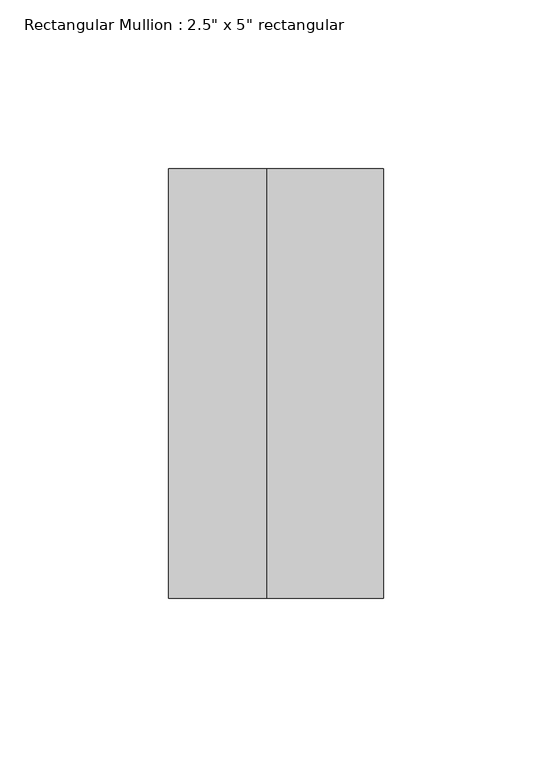
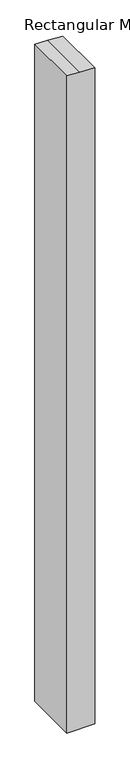
"""IFC4 building model written with IfcOpenShell, lengths in millimetres: member geometry."""

import ifcopenshell
import ifcopenshell.guid

model = None  # the IFC model being written
_history = None  # IfcOwnerHistory: only IFC2X3 demands one
_inside = {}  # id of a spatial element -> (the spatial element, [elements in it])
_under = {}  # id of a project, library or spatial element -> (it, [spatial elements below it])
_declared = {}  # id of a project -> (the project, [libraries it declares])
_typed = {}  # id of a type object -> (the type object, [elements of that type])
_made_of = {}  # id of a material, layer set ... -> (it, [elements and type objects made of it])


def new_model(schema):
    """Start an empty IFC model of exactly this schema.

    Asked for "IFC4X3", IfcOpenShell would pick the latest addendum, in which some entities
    have other attributes; the version numbers below select the first issue.
    IFC2X3 requires an IfcOwnerHistory on every rooted entity: one is made here for all.
    """
    global model, _history
    if schema == "IFC4X3":
        model = ifcopenshell.file(schema_version=(4, 3, 0, 0))
    else:
        model = ifcopenshell.file(schema=schema)
    _inside.clear()
    _under.clear()
    _declared.clear()
    _typed.clear()
    _made_of.clear()
    _history = None
    if model.schema == "IFC2X3":
        org = make("IfcOrganization", Name="unknown")
        user = make(
            "IfcPersonAndOrganization",
            ThePerson=make("IfcPerson", FamilyName="unknown"),
            TheOrganization=org,
        )
        app = make(
            "IfcApplication",
            ApplicationDeveloper=org,
            Version="unknown",
            ApplicationFullName="unknown",
            ApplicationIdentifier="unknown",
        )
        _history = make(
            "IfcOwnerHistory",
            OwningUser=user,
            OwningApplication=app,
            ChangeAction="ADDED",
            CreationDate=0,
        )
    return model


def make(cls, **values):
    """One entity of the class cls with the attributes given. An attribute that is None is left unset."""
    return model.create_entity(
        cls, **{name: value for name, value in values.items() if value is not None}
    )


def rooted(cls, **values):
    """An entity with a GlobalId (a new one), such as an element, a storey or a relation."""
    return make(cls, GlobalId=ifcopenshell.guid.new(), OwnerHistory=_history, **values)


def si_unit(unit_type, name, prefix=None):
    """IfcSIUnit, for example si_unit("LENGTHUNIT", "METRE", prefix="MILLI")."""
    return make("IfcSIUnit", UnitType=unit_type, Prefix=prefix, Name=name)


def assignment(units):
    """IfcUnitAssignment: the units of a project."""
    return None if units is None else make("IfcUnitAssignment", Units=units)


def point(xyz):
    """IfcCartesianPoint."""
    return None if xyz is None else make("IfcCartesianPoint", Coordinates=xyz)


def direction(xyz):
    """IfcDirection."""
    return None if xyz is None else make("IfcDirection", DirectionRatios=xyz)


def frame(location, z_axis=None, x_axis=None):
    """IfcAxis2Placement3D, a coordinate frame: its origin and axes. An axis left out is left unset."""
    return make(
        "IfcAxis2Placement3D",
        Location=point(location),
        Axis=direction(z_axis),
        RefDirection=direction(x_axis),
    )


def origin():
    """The frame at (0, 0, 0) with its axes left unset."""
    return frame((0.0, 0.0, 0.0))


def place(relative_to, where):
    """IfcLocalPlacement: puts the frame where relative to a parent placement (None: the world)."""
    return make(
        "IfcLocalPlacement", PlacementRelTo=relative_to, RelativePlacement=where
    )


def context(
    kind, dimensions, precision=None, world=None, true_north=None, identifier=None
):
    """IfcGeometricRepresentationContext, for example the 3D "Model" context."""
    return make(
        "IfcGeometricRepresentationContext",
        ContextIdentifier=identifier,
        ContextType=kind,
        CoordinateSpaceDimension=dimensions,
        Precision=precision,
        WorldCoordinateSystem=world,
        TrueNorth=true_north,
    )


def project(units=None, contexts=None):
    """IfcProject with its units and contexts."""
    return rooted(
        "IfcProject",
        Name="project",
        RepresentationContexts=contexts,
        UnitsInContext=assignment(units),
    )


def spatial(cls, under=None, at=None, **own):
    """A site, building, storey or space (cls), placed at a placement, below another one or the project."""
    s = rooted(cls, ObjectPlacement=at, **own)
    if under is not None:
        _under.setdefault(under.id(), (under, []))[1].append(s)
    return s


def polyline(points):
    """IfcPolyline through the points."""
    return make("IfcPolyline", Points=[point(p) for p in points])


def outline(outer, holes=None, kind="AREA"):
    """IfcArbitraryClosedProfileDef: a profile drawn as a closed curve; with holes, ...WithVoids."""
    if holes is None:
        return make("IfcArbitraryClosedProfileDef", ProfileType=kind, OuterCurve=outer)
    return make(
        "IfcArbitraryProfileDefWithVoids",
        ProfileType=kind,
        OuterCurve=outer,
        InnerCurves=holes,
    )


def extrude(swept, where, along, depth):
    """IfcExtrudedAreaSolid: the profile swept, set in the frame where, extruded along a direction by depth."""
    return make(
        "IfcExtrudedAreaSolid",
        SweptArea=swept,
        Position=where,
        ExtrudedDirection=direction(along),
        Depth=depth,
    )


def shape(context_of_items, identifier, shape_type, items):
    """IfcShapeRepresentation: the items that make up one representation, for example the "Body"."""
    return make(
        "IfcShapeRepresentation",
        ContextOfItems=context_of_items,
        RepresentationIdentifier=identifier,
        RepresentationType=shape_type,
        Items=items,
    )


def source(mapping_origin, context_of_items, identifier, shape_type, items):
    """IfcRepresentationMap: a shape defined once, which mapped items show again and again."""
    return make(
        "IfcRepresentationMap",
        MappingOrigin=mapping_origin,
        MappedRepresentation=shape(context_of_items, identifier, shape_type, items),
    )


def transform(
    local_origin,
    x_axis=None,
    y_axis=None,
    z_axis=None,
    scale=None,
    scale2=None,
    scale3=None,
    uniform=True,
):
    """IfcCartesianTransformationOperator3D, or its non-uniform kind. x_axis, y_axis, z_axis: its Axis1, 2, 3."""
    if uniform:
        return make(
            "IfcCartesianTransformationOperator3D",
            Axis1=direction(x_axis),
            Axis2=direction(y_axis),
            LocalOrigin=point(local_origin),
            Scale=scale,
            Axis3=direction(z_axis),
        )
    return make(
        "IfcCartesianTransformationOperator3DnonUniform",
        Axis1=direction(x_axis),
        Axis2=direction(y_axis),
        LocalOrigin=point(local_origin),
        Scale=scale,
        Axis3=direction(z_axis),
        Scale2=scale2,
        Scale3=scale3,
    )


def mapped(mapping_source, mapping_target):
    """IfcMappedItem: shows the shape of a source again, moved by a transform."""
    return make(
        "IfcMappedItem", MappingSource=mapping_source, MappingTarget=mapping_target
    )


def made_of(thing, what):
    """Note that an element or type object is made of a material, layer set ...; save() writes the relation."""
    if what is not None:
        _made_of.setdefault(what.id(), (what, []))[1].append(thing)
    return thing


def element(
    cls,
    number,
    at=None,
    inside=None,
    cuts=None,
    type_object=None,
    material=None,
    context=None,
    identifier="Body",
    shape_type=None,
    held_by="IfcProductDefinitionShape",
    body=None,
    shapes=None,
    **own,
):
    """One element of the class cls, such as IfcWall. Its Tag is "e" and its number.

    at: its placement. inside: the storey or other place that contains it. cuts: it is an
    opening in that element (IfcRelVoidsElement). A single representation is given by context,
    identifier, shape_type and body (its items); several are given by shapes. held_by: the class
    of the entity that holds the representations. save() writes the other relations.
    """
    e = rooted(cls, Tag="e%d" % number, ObjectPlacement=at, **own)
    if body is not None:
        shapes = [shape(context, identifier, shape_type, body)]
    if shapes is not None:
        e.Representation = make(held_by, Representations=shapes)
    if inside is not None:
        _inside.setdefault(inside.id(), (inside, []))[1].append(e)
    if cuts is not None:
        rooted(
            "IfcRelVoidsElement", RelatingBuildingElement=cuts, RelatedOpeningElement=e
        )
    if type_object is not None:
        _typed.setdefault(type_object.id(), (type_object, []))[1].append(e)
    return made_of(e, material)


def aggregate(whole, parts):
    """IfcRelAggregates: a whole, such as a stair, and the parts it consists of."""
    return rooted("IfcRelAggregates", RelatingObject=whole, RelatedObjects=parts)


def save(model, path):
    """Write the relations noted so far, then the file.

    IfcRelAggregates (storeys below a building ...), IfcRelContainedInSpatialStructure (elements
    in a storey), IfcRelDefinesByType, IfcRelAssociatesMaterial and IfcRelDeclares: one each for
    every whole, place, type object, material and project.
    """
    for whole, parts in _under.values():
        aggregate(whole, parts)
    for where, things in _inside.values():
        rooted(
            "IfcRelContainedInSpatialStructure",
            RelatedElements=things,
            RelatingStructure=where,
        )
    for kind, things in _typed.values():
        rooted("IfcRelDefinesByType", RelatedObjects=things, RelatingType=kind)
    for what, things in _made_of.values():
        rooted("IfcRelAssociatesMaterial", RelatedObjects=things, RelatingMaterial=what)
    for by, libraries in _declared.values():
        rooted("IfcRelDeclares", RelatingContext=by, RelatedDefinitions=libraries)
    model.write(path)


def member_542ec671(model_context):
    return source(origin(), model_context, "Body", "SweptSolid", [
        extrude(outline(polyline([(-64.8775557, 31.75), (-63.4449853, -2.6426951), (-62.232569, -31.75), (-1651.5778232, -31.75), (-1651.5778232, 31.75), (-64.8775557, 31.75)])), frame((0.0, -63.5, 0.0), z_axis=(0.0, 1.0, 0.0), x_axis=(0.0, 0.0, 1.0)), (0.0, 0.0, 1.0), 127.0),
    ])


if __name__ == "__main__":
    model = new_model("IFC4")
    model_context = context("Model", 3, world=origin())
    ifc_project = project(units=[si_unit("LENGTHUNIT", "METRE", prefix="MILLI")], contexts=[model_context])
    site = spatial("IfcSite", under=ifc_project)
    building = spatial("IfcBuilding", under=site)
    placement = place(None, origin())
    member_shape = member_542ec671(model_context)
    element("IfcMember", 1, ObjectType="Rectangular Mullion : 2.5\" x 5\" rectangular", at=placement, inside=building, context=model_context, shape_type="MappedRepresentation", body=[
        mapped(member_shape, transform((0.0, 0.0, 0.0), x_axis=(1.0, 0.0, 0.0), y_axis=(0.0, 1.0, 0.0), z_axis=(0.0, 0.0, 1.0))),
    ])
    save(model, "model.ifc")

# Revit data of these elements
# Project information
#   Organization Name = "Gannett Fleming, Inc."
#   Building Name = "Health Center"
#   Design Option = "Main Model"
#   Project Issue Date = "April 1, 2021"
#   Project Status = "04-01-21 ARCHITECTURAL CHECK SET"
#   Client Name = "Autodesk"
#   Project Address = "Enter address here"
#   Project Name = "Revit 2021\nDataset Model"
#   Project Number = "056750"
# Type "Rectangular Mullion : 2.5\" x 5\" rectangular"
#   built-in parameter 1007304 = 0.416667 (stored number, unit not read)
#   built-in parameter 1007301 = 0.104167 (stored number, unit not read)
#   built-in parameter 1007300 = 0.104167 (stored number, unit not read)
# Element 1 (IfcMember, "Rectangular Mullion : 2.5\" x 5\" rectangular")
#   Materials on its faces: "Aluminum"
# Materials
#   "Aluminum": class "Metal", colour RGB 247 247 247, transparency 0, Description = "Aluminum 6061", Cost = 0
